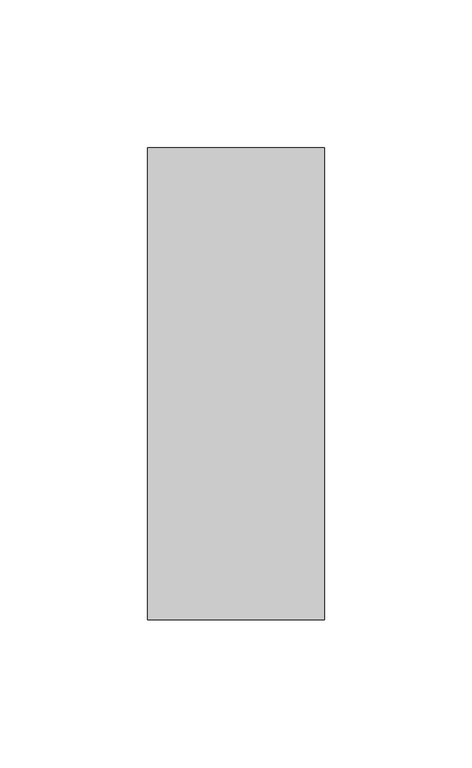
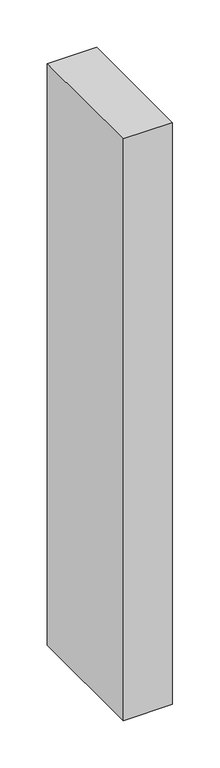
"""IFC4 building model written with IfcOpenShell, lengths in millimetres: column geometry, Madeira de lei-Coluna : Pontalete 6X16cm."""

from ifc_helpers import new_model, si_unit, frame, origin, place, context, project, spatial, polyline, outline, extrude, source, transform, mapped, element, save


def column_d505325c(model_context):
    return source(origin(), model_context, "Body", "SweptSolid", [
        extrude(outline(polyline([(30.0, 80.0), (30.0, -80.0), (-30.0, -80.0), (-30.0, 80.0), (30.0, 80.0)])), frame((0.0, 0.0, 6710.0), z_axis=(0.0, 0.0, 1.0), x_axis=(1.0, 0.0, 0.0)), (0.0, 0.0, 1.0), 750.0),
    ])


if __name__ == "__main__":
    model = new_model("IFC4")
    model_context = context("Model", 3, world=origin())
    ifc_project = project(units=[si_unit("LENGTHUNIT", "METRE", prefix="MILLI")], contexts=[model_context])
    site = spatial("IfcSite", under=ifc_project)
    building = spatial("IfcBuilding", under=site)
    placement = place(None, origin())
    column_shape = column_d505325c(model_context)
    element("IfcColumn", 1, ObjectType="Madeira de lei-Coluna : Pontalete 6X16cm", at=placement, inside=building, context=model_context, shape_type="MappedRepresentation", body=[
        mapped(column_shape, transform((0.0, 0.0, 0.0), x_axis=(1.0, 0.0, 0.0), y_axis=(0.0, 1.0, 0.0), z_axis=(0.0, 0.0, 1.0))),
    ])
    save(model, "model.ifc")

# Revit data of these elements
# Type "Madeira de lei-Coluna : Pontalete 6X16cm"
#   A = 0.01952 m²
#   b = 0.06 m
#   d = 0.16 m
#   Structural Material [instance default] = none
#   Assembly Code = ""
# Element 1 (IfcColumn, "Madeira de lei-Coluna : Pontalete 6X16cm")
#   Structural Material = .MADEIRAMENTO
#   Materials on its faces: ".MADEIRAMENTO"
# Materials
#   ".MADEIRAMENTO": class ".CC_MADEIRAS", colour RGB 212 179 113, transparency 0, Cost = 0
